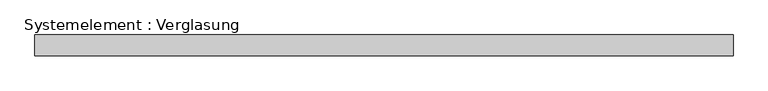
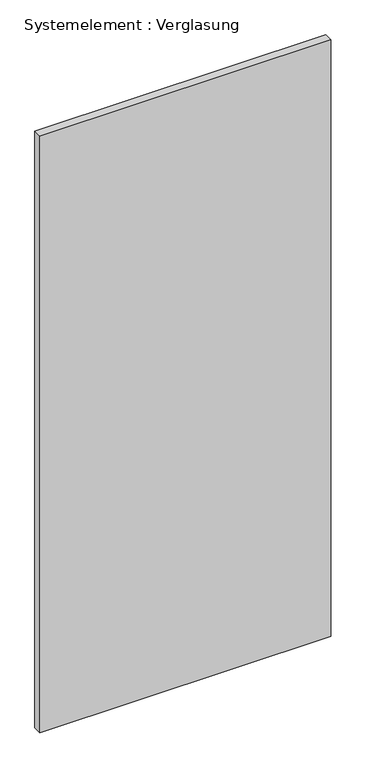
"""IFC4 building model written with IfcOpenShell, lengths in millimetres: plate geometry, Systemelement : Verglasung."""

from ifc_helpers import new_model, si_unit, origin, origin_with_axes, place, context, project, spatial, polyline, outline, extrude, source, transform, mapped, element, save


def systemelement_verglasung_22fa5f51(model_context):
    return source(origin(), model_context, "Body", "SweptSolid", [
        extrude(outline(polyline([(504.9886524, -15.0), (-504.9886524, -15.0), (-504.9886524, 15.0), (504.9886524, 15.0), (504.9886524, -15.0)])), origin_with_axes(), (0.0, 0.0, 1.0), 2190.0),
    ])


if __name__ == "__main__":
    model = new_model("IFC4")
    model_context = context("Model", 3, world=origin())
    ifc_project = project(units=[si_unit("LENGTHUNIT", "METRE", prefix="MILLI")], contexts=[model_context])
    site = spatial("IfcSite", under=ifc_project)
    building = spatial("IfcBuilding", under=site)
    placement = place(None, origin())
    systemelement_verglasung_shape = systemelement_verglasung_22fa5f51(model_context)
    element("IfcPlate", 1, ObjectType="Systemelement : Verglasung", at=placement, inside=building, context=model_context, shape_type="MappedRepresentation", body=[
        mapped(systemelement_verglasung_shape, transform((0.0, 0.0, 0.0), x_axis=(1.0, 0.0, 0.0), y_axis=(0.0, 1.0, 0.0), z_axis=(0.0, 0.0, 1.0))),
    ])
    save(model, "model.ifc")

# Revit data of these elements
# Type "Systemelement : Verglasung"
#   Construction Type Id = "GSP4R"
#   Analytic Construction = "1/8 Zoll Pilkington-Verglasung einfach"
#   Visual Light Transmittance = 0.9
#   Solar Heat Gain Coefficient = 0.86
#   Heat Transfer Coefficient (U) = 6.7069 W/(m²·K)
# Element 1 (IfcPlate, "Systemelement : Verglasung")
#   Materials on its faces: "Glas"
# Materials
#   "Glas": class "Glas", colour RGB 0 0 255, transparency 0.75, Comments = "Render-Darstellung nicht aktualisiert ", Cost = 0
